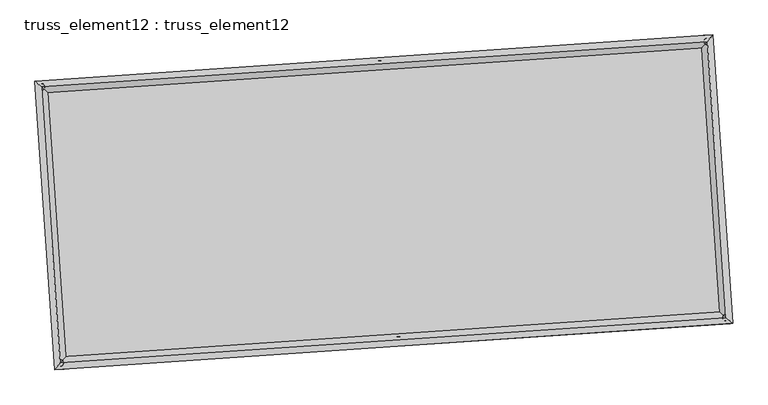
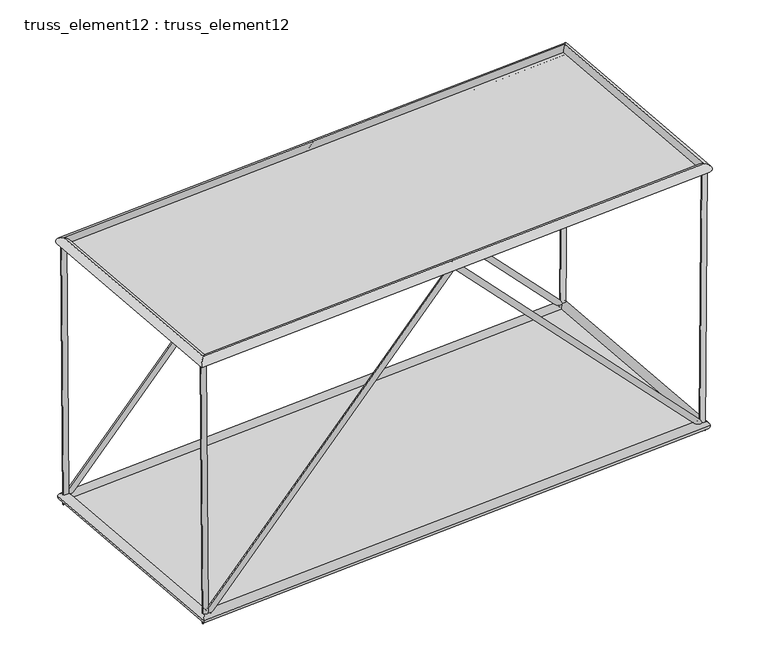
"""IFC4 building model written with IfcOpenShell, lengths in millimetres: plate geometry, truss_element12 : truss_element12."""

import ifcopenshell
import ifcopenshell.guid

model = None  # the IFC model being written
_history = None  # IfcOwnerHistory: only IFC2X3 demands one
_inside = {}  # id of a spatial element -> (the spatial element, [elements in it])
_under = {}  # id of a project, library or spatial element -> (it, [spatial elements below it])
_declared = {}  # id of a project -> (the project, [libraries it declares])
_typed = {}  # id of a type object -> (the type object, [elements of that type])
_made_of = {}  # id of a material, layer set ... -> (it, [elements and type objects made of it])


def new_model(schema):
    """Start an empty IFC model of exactly this schema.

    Asked for "IFC4X3", IfcOpenShell would pick the latest addendum, in which some entities
    have other attributes; the version numbers below select the first issue.
    IFC2X3 requires an IfcOwnerHistory on every rooted entity: one is made here for all.
    """
    global model, _history
    if schema == "IFC4X3":
        model = ifcopenshell.file(schema_version=(4, 3, 0, 0))
    else:
        model = ifcopenshell.file(schema=schema)
    _inside.clear()
    _under.clear()
    _declared.clear()
    _typed.clear()
    _made_of.clear()
    _history = None
    if model.schema == "IFC2X3":
        org = make("IfcOrganization", Name="unknown")
        user = make(
            "IfcPersonAndOrganization",
            ThePerson=make("IfcPerson", FamilyName="unknown"),
            TheOrganization=org,
        )
        app = make(
            "IfcApplication",
            ApplicationDeveloper=org,
            Version="unknown",
            ApplicationFullName="unknown",
            ApplicationIdentifier="unknown",
        )
        _history = make(
            "IfcOwnerHistory",
            OwningUser=user,
            OwningApplication=app,
            ChangeAction="ADDED",
            CreationDate=0,
        )
    return model


def make(cls, **values):
    """One entity of the class cls with the attributes given. An attribute that is None is left unset."""
    return model.create_entity(
        cls, **{name: value for name, value in values.items() if value is not None}
    )


def rooted(cls, **values):
    """An entity with a GlobalId (a new one), such as an element, a storey or a relation."""
    return make(cls, GlobalId=ifcopenshell.guid.new(), OwnerHistory=_history, **values)


def si_unit(unit_type, name, prefix=None):
    """IfcSIUnit, for example si_unit("LENGTHUNIT", "METRE", prefix="MILLI")."""
    return make("IfcSIUnit", UnitType=unit_type, Prefix=prefix, Name=name)


def assignment(units):
    """IfcUnitAssignment: the units of a project."""
    return None if units is None else make("IfcUnitAssignment", Units=units)


def point(xyz):
    """IfcCartesianPoint."""
    return None if xyz is None else make("IfcCartesianPoint", Coordinates=xyz)


def direction(xyz):
    """IfcDirection."""
    return None if xyz is None else make("IfcDirection", DirectionRatios=xyz)


def frame(location, z_axis=None, x_axis=None):
    """IfcAxis2Placement3D, a coordinate frame: its origin and axes. An axis left out is left unset."""
    return make(
        "IfcAxis2Placement3D",
        Location=point(location),
        Axis=direction(z_axis),
        RefDirection=direction(x_axis),
    )


def origin():
    """The frame at (0, 0, 0) with its axes left unset."""
    return frame((0.0, 0.0, 0.0))


def origin_with_axes():
    """The frame at (0, 0, 0) with the z axis (0, 0, 1) and the x axis (1, 0, 0) written out."""
    return frame((0.0, 0.0, 0.0), z_axis=(0.0, 0.0, 1.0), x_axis=(1.0, 0.0, 0.0))


def place(relative_to, where):
    """IfcLocalPlacement: puts the frame where relative to a parent placement (None: the world)."""
    return make(
        "IfcLocalPlacement", PlacementRelTo=relative_to, RelativePlacement=where
    )


def context(
    kind, dimensions, precision=None, world=None, true_north=None, identifier=None
):
    """IfcGeometricRepresentationContext, for example the 3D "Model" context."""
    return make(
        "IfcGeometricRepresentationContext",
        ContextIdentifier=identifier,
        ContextType=kind,
        CoordinateSpaceDimension=dimensions,
        Precision=precision,
        WorldCoordinateSystem=world,
        TrueNorth=true_north,
    )


def project(units=None, contexts=None):
    """IfcProject with its units and contexts."""
    return rooted(
        "IfcProject",
        Name="project",
        RepresentationContexts=contexts,
        UnitsInContext=assignment(units),
    )


def spatial(cls, under=None, at=None, **own):
    """A site, building, storey or space (cls), placed at a placement, below another one or the project."""
    s = rooted(cls, ObjectPlacement=at, **own)
    if under is not None:
        _under.setdefault(under.id(), (under, []))[1].append(s)
    return s


def polyline(points):
    """IfcPolyline through the points."""
    return make("IfcPolyline", Points=[point(p) for p in points])


def circle_curve(where, radius):
    """IfcCircle in the frame where."""
    return make("IfcCircle", Position=where, Radius=radius)


def ellipse_curve(where, semi_axis1, semi_axis2):
    """IfcEllipse in the frame where."""
    return make(
        "IfcEllipse", Position=where, SemiAxis1=semi_axis1, SemiAxis2=semi_axis2
    )


def outline(outer, holes=None, kind="AREA"):
    """IfcArbitraryClosedProfileDef: a profile drawn as a closed curve; with holes, ...WithVoids."""
    if holes is None:
        return make("IfcArbitraryClosedProfileDef", ProfileType=kind, OuterCurve=outer)
    return make(
        "IfcArbitraryProfileDefWithVoids",
        ProfileType=kind,
        OuterCurve=outer,
        InnerCurves=holes,
    )


def extrude(swept, where, along, depth):
    """IfcExtrudedAreaSolid: the profile swept, set in the frame where, extruded along a direction by depth."""
    return make(
        "IfcExtrudedAreaSolid",
        SweptArea=swept,
        Position=where,
        ExtrudedDirection=direction(along),
        Depth=depth,
    )


def shape(context_of_items, identifier, shape_type, items):
    """IfcShapeRepresentation: the items that make up one representation, for example the "Body"."""
    return make(
        "IfcShapeRepresentation",
        ContextOfItems=context_of_items,
        RepresentationIdentifier=identifier,
        RepresentationType=shape_type,
        Items=items,
    )


def source(mapping_origin, context_of_items, identifier, shape_type, items):
    """IfcRepresentationMap: a shape defined once, which mapped items show again and again."""
    return make(
        "IfcRepresentationMap",
        MappingOrigin=mapping_origin,
        MappedRepresentation=shape(context_of_items, identifier, shape_type, items),
    )


def transform(
    local_origin,
    x_axis=None,
    y_axis=None,
    z_axis=None,
    scale=None,
    scale2=None,
    scale3=None,
    uniform=True,
):
    """IfcCartesianTransformationOperator3D, or its non-uniform kind. x_axis, y_axis, z_axis: its Axis1, 2, 3."""
    if uniform:
        return make(
            "IfcCartesianTransformationOperator3D",
            Axis1=direction(x_axis),
            Axis2=direction(y_axis),
            LocalOrigin=point(local_origin),
            Scale=scale,
            Axis3=direction(z_axis),
        )
    return make(
        "IfcCartesianTransformationOperator3DnonUniform",
        Axis1=direction(x_axis),
        Axis2=direction(y_axis),
        LocalOrigin=point(local_origin),
        Scale=scale,
        Axis3=direction(z_axis),
        Scale2=scale2,
        Scale3=scale3,
    )


def mapped(mapping_source, mapping_target):
    """IfcMappedItem: shows the shape of a source again, moved by a transform."""
    return make(
        "IfcMappedItem", MappingSource=mapping_source, MappingTarget=mapping_target
    )


def made_of(thing, what):
    """Note that an element or type object is made of a material, layer set ...; save() writes the relation."""
    if what is not None:
        _made_of.setdefault(what.id(), (what, []))[1].append(thing)
    return thing


def element(
    cls,
    number,
    at=None,
    inside=None,
    cuts=None,
    type_object=None,
    material=None,
    context=None,
    identifier="Body",
    shape_type=None,
    held_by="IfcProductDefinitionShape",
    body=None,
    shapes=None,
    **own,
):
    """One element of the class cls, such as IfcWall. Its Tag is "e" and its number.

    at: its placement. inside: the storey or other place that contains it. cuts: it is an
    opening in that element (IfcRelVoidsElement). A single representation is given by context,
    identifier, shape_type and body (its items); several are given by shapes. held_by: the class
    of the entity that holds the representations. save() writes the other relations.
    """
    e = rooted(cls, Tag="e%d" % number, ObjectPlacement=at, **own)
    if body is not None:
        shapes = [shape(context, identifier, shape_type, body)]
    if shapes is not None:
        e.Representation = make(held_by, Representations=shapes)
    if inside is not None:
        _inside.setdefault(inside.id(), (inside, []))[1].append(e)
    if cuts is not None:
        rooted(
            "IfcRelVoidsElement", RelatingBuildingElement=cuts, RelatedOpeningElement=e
        )
    if type_object is not None:
        _typed.setdefault(type_object.id(), (type_object, []))[1].append(e)
    return made_of(e, material)


def aggregate(whole, parts):
    """IfcRelAggregates: a whole, such as a stair, and the parts it consists of."""
    return rooted("IfcRelAggregates", RelatingObject=whole, RelatedObjects=parts)


def save(model, path):
    """Write the relations noted so far, then the file.

    IfcRelAggregates (storeys below a building ...), IfcRelContainedInSpatialStructure (elements
    in a storey), IfcRelDefinesByType, IfcRelAssociatesMaterial and IfcRelDeclares: one each for
    every whole, place, type object, material and project.
    """
    for whole, parts in _under.values():
        aggregate(whole, parts)
    for where, things in _inside.values():
        rooted(
            "IfcRelContainedInSpatialStructure",
            RelatedElements=things,
            RelatingStructure=where,
        )
    for kind, things in _typed.values():
        rooted("IfcRelDefinesByType", RelatedObjects=things, RelatingType=kind)
    for what, things in _made_of.values():
        rooted("IfcRelAssociatesMaterial", RelatedObjects=things, RelatingMaterial=what)
    for by, libraries in _declared.values():
        rooted("IfcRelDeclares", RelatingContext=by, RelatedDefinitions=libraries)
    model.write(path)


def plane_surface(at):
    """IfcPlane: the flat surface through the origin of the frame at, square to its z axis."""
    return make("IfcPlane", Position=at)


def cylinder_surface(at, radius):
    """IfcCylindricalSurface: all points at the distance radius from the z axis of the frame at."""
    return make("IfcCylindricalSurface", Position=at, Radius=radius)


def advanced_brep(points, edges, surfaces, faces):
    """IfcAdvancedBrep: a solid bounded by faces that lie on surfaces and meet in shared edges.

    An edge is (start, end): straight between two places in points (the first is 0);
    or (start, end, curve); or (start, end, curve, False) where it runs against its curve.
    A face is (place in surfaces, loops), or (place, loops, False) where it looks against
    its surface's normal. A loop lists edges by number (the first is 1), with a minus sign
    where the edge is run from its end to its start. The first loop is the outer one.
    """
    corners = [point(p) for p in points]
    vertices = [make("IfcVertexPoint", VertexGeometry=c) for c in corners]
    made = []
    for start, end, *more in edges:
        made.append(
            make(
                "IfcEdgeCurve",
                EdgeStart=vertices[start],
                EdgeEnd=vertices[end],
                EdgeGeometry=more[0] if more else make("IfcPolyline", Points=[corners[start], corners[end]]),
                SameSense=more[1] if len(more) > 1 else True,
            )
        )
    hull = []
    for where, loops, *sense in faces:
        bounds = []
        for j, loop in enumerate(loops):
            ring = [make("IfcOrientedEdge", EdgeElement=made[abs(k) - 1], Orientation=k > 0) for k in loop]
            bounds.append(
                make(
                    "IfcFaceOuterBound" if j == 0 else "IfcFaceBound",
                    Bound=make("IfcEdgeLoop", EdgeList=ring),
                    Orientation=True,
                )
            )
        hull.append(make("IfcAdvancedFace", Bounds=bounds, FaceSurface=surfaces[where], SameSense=sense[0] if sense else True))
    return make("IfcAdvancedBrep", Outer=make("IfcClosedShell", CfsFaces=hull))


def truss_element12_truss_element12_81932074(model_context):
    return source(origin(), model_context, "Body", "SolidModel", [
        advanced_brep(
        [(-3702.688172, 2273.6501932, 5000.2343714), (-3801.788684, 2260.2891126, 4999.4793629), (-3665.8706913, 2276.1606372, 123.2387715), (-3763.1161915, 2262.9260429, -123.2387715), (1063.4172149, 2598.6328018, 5071.9820194), (1063.8699312, 2592.0598775, 4927.7362286), (5793.2948238, 2921.145176, 123.2430249), (5891.4661532, 2921.2353125, -123.2430249), (5829.5270694, 2923.6157151, 5000.2328852), (5929.5240788, 2923.8303377, 4999.4898764)],
        [
            (0, 1, circle_curve(frame((-3752.238428, 2266.9696529, 4999.8568672), z_axis=(-0.007548997314577087, -0.000514737430455595, 0.999971373432721), x_axis=(-0.13361086689497337, 0.9910337470163174, -0.0004985201818760374)), 50.0)),
            (1, 0, circle_curve(frame((-3752.238428, 2266.9696529, 4999.8568672), z_axis=(-0.007548997314577087, -0.000514737430455595, 0.999971373432721), x_axis=(-0.13361086689497337, 0.9910337470163174, -0.0004985201818760374)), 50.0)),
            (0, 2),
            (2, 3, ellipse_curve(frame((-3714.4934414, 2269.54334, 0.0), z_axis=(-0.9271929359308112, -0.06322176171080186, 0.36921033084975474), x_axis=(0.36835501674811216, 0.025116728343544507, 0.9293458622029878)), 132.8968359, 50.0)),
            (3, 1),
            (3, 2, ellipse_curve(frame((-3714.4934414, 2269.54334, 0.0), z_axis=(-0.9271929359308112, -0.06322176171080186, 0.36921033084975474), x_axis=(0.36835501674811216, 0.025116728343544507, 0.9293458622029878)), 132.8968359, 50.0)),
            (2, 4),
            (4, 5, ellipse_curve(frame((1063.6435731, 2595.3463397, 4999.859124), z_axis=(-0.9976833955843888, -0.06802823819525586, -3.135687396447292e-05), x_axis=(3.12842325072798e-05, 2.133152891987861e-06, -0.9999999995083733)), 72.2799434, 50.0)),
            (5, 3),
            (5, 4, ellipse_curve(frame((1063.6435731, 2595.3463397, 4999.859124), z_axis=(-0.9976833955843888, -0.06802823819525586, -3.135687396447292e-05), x_axis=(3.12842325072798e-05, 2.133152891987861e-06, -0.9999999995083733)), 72.2799434, 50.0)),
            (4, 6),
            (6, 7, ellipse_curve(frame((5842.3804885, 2921.1902443, 0.0), z_axis=(-0.9271592320010842, -0.06321946356795421, -0.36929535326258833), x_axis=(-0.36843984219769044, -0.025122512268499313, 0.9293120800133075)), 132.9062538, 50.0)),
            (7, 5),
            (7, 6, ellipse_curve(frame((5842.3804885, 2921.1902443, 0.0), z_axis=(-0.9271592320010842, -0.06321946356795421, -0.36929535326258833), x_axis=(-0.36843984219769044, -0.025122512268499313, 0.9293120800133075)), 132.9062538, 50.0)),
            (8, 9, circle_curve(frame((5879.5255741, 2923.7230264, 4999.8613808), z_axis=(0.007429017120522426, 0.0005065564371105527, 0.9999722761682942), x_axis=(-0.0021499302803911083, 0.999997568554261, -0.0004905969378120464)), 50.0)),
            (9, 8, circle_curve(frame((5879.5255741, 2923.7230264, 4999.8613808), z_axis=(0.007429017120522426, 0.0005065564371105527, 0.9999722761682942), x_axis=(-0.0021499302803911083, 0.999997568554261, -0.0004905969378120464)), 50.0)),
            (6, 8),
            (9, 7),
        ],
        [
            plane_surface(frame((-3752.238428, 2316.9696463, 4999.8826048), z_axis=(-0.007548997314575647, -0.0005147374304560255, 0.9999713734327211), x_axis=(0.9999715059138159, -3.885862204455747e-06, 0.007548996314447718))),
            cylinder_surface(frame((-3752.238428, 2266.9696529, 4999.8568672), z_axis=(-0.007548997314577087, -0.000514737430455595, 0.999971373432721), x_axis=(-0.13361086689497337, 0.9910337470163174, -0.0004985201818760374)), 50.0),
            cylinder_surface(frame((-3714.4934414, 2269.54334, 0.0), z_axis=(-0.6901297168790946, -0.04705732196532738, -0.7221541264368931), x_axis=(-0.02041156189161515, 0.9987523773136525, -0.04557474027871566)), 50.0),
            cylinder_surface(frame((1063.6435731, 2595.3463397, 4999.859124), z_axis=(-0.6901748995971223, -0.04706040280311382, 0.7221107438988223), x_axis=(-0.115346442987764, 0.9922791286529746, -0.04557772405203943)), 50.0),
            plane_surface(frame((5879.5255741, 2873.7230329, 4999.8867094), z_axis=(0.007429017120522355, 0.0005065564371127904, 0.9999722761682942), x_axis=(0.999972404471555, -3.7633202953912764e-06, -0.0074290161673289294))),
            cylinder_surface(frame((5842.3804885, 2921.1902443, 0.0), z_axis=(-0.007429017120522424, -0.0005065564371105526, -0.999972276168294), x_axis=(-0.0021499302803911083, 0.999997568554261, -0.0004905969378120464)), 50.0),
        ],
        [
            (0, [[1, 2]]),
            (1, [[-1, 3, 4, 5]]),
            (1, [[-2, -5, 6, -3]]),
            (2, [[-4, 7, 8, 9]]),
            (2, [[-6, -9, 10, -7]]),
            (3, [[-8, 11, 12, 13]]),
            (3, [[-10, -13, 14, -11]]),
            (4, [[15, 16]]),
            (5, [[-12, 17, -16, 18]]),
            (5, [[-14, -18, -15, -17]]),
        ],
    ),
        advanced_brep(
        [(-3430.575219, -1717.0833911, 5000.2343714), (-3529.6757311, -1730.4444717, 4999.4793629), (-3393.7577384, -1714.5729471, 123.2387715), (-3491.0032386, -1727.8075414, -123.2387715), (1335.5301678, -1392.1007825, 5071.9820194), (1335.9828841, -1398.6737068, 4927.7362286), (6065.4077767, -1069.5884083, 123.2430249), (6163.5791061, -1069.4982718, -123.2430249), (6101.6400224, -1067.1178692, 5000.2328852), (6201.6370317, -1066.9032466, 4999.4898764)],
        [
            (0, 1, circle_curve(frame((-3480.1254751, -1723.7639314, 4999.8568672), z_axis=(-0.00754899731457709, -0.0005147374304555873, 0.999971373432721), x_axis=(-0.13361086689497323, 0.9910337470163173, -0.0004985201818760446)), 50.0)),
            (1, 0, circle_curve(frame((-3480.1254751, -1723.7639314, 4999.8568672), z_axis=(-0.00754899731457709, -0.0005147374304555873, 0.999971373432721), x_axis=(-0.13361086689497323, 0.9910337470163173, -0.0004985201818760446)), 50.0)),
            (0, 2),
            (2, 3, ellipse_curve(frame((-3442.3804885, -1721.1902443, 0.0), z_axis=(-0.9271929359308112, -0.06322176171080175, 0.3692103308497547), x_axis=(0.3683550167481121, 0.025116728343544472, 0.9293458622029878)), 132.8968359, 50.0)),
            (3, 1),
            (3, 2, ellipse_curve(frame((-3442.3804885, -1721.1902443, 0.0), z_axis=(-0.9271929359308112, -0.06322176171080175, 0.3692103308497547), x_axis=(0.3683550167481121, 0.025116728343544472, 0.9293458622029878)), 132.8968359, 50.0)),
            (2, 4),
            (4, 5, ellipse_curve(frame((1335.756526, -1395.3872446, 4999.859124), z_axis=(-0.9976833955843888, -0.06802823819525583, -3.135687396431242e-05), x_axis=(3.1284232507126054e-05, 2.1331528920551236e-06, -0.9999999995083733)), 72.2799434, 50.0)),
            (5, 3),
            (5, 4, ellipse_curve(frame((1335.756526, -1395.3872446, 4999.859124), z_axis=(-0.9976833955843888, -0.06802823819525583, -3.135687396431242e-05), x_axis=(3.1284232507126054e-05, 2.1331528920551236e-06, -0.9999999995083733)), 72.2799434, 50.0)),
            (4, 6),
            (6, 7, ellipse_curve(frame((6114.4934414, -1069.54334, 0.0), z_axis=(-0.9271592320010842, -0.06321946356795434, -0.3692953532625882), x_axis=(-0.3684398421976903, -0.025122512268499313, 0.9293120800133076)), 132.9062538, 50.0)),
            (7, 5),
            (7, 6, ellipse_curve(frame((6114.4934414, -1069.54334, 0.0), z_axis=(-0.9271592320010842, -0.06321946356795434, -0.3692953532625882), x_axis=(-0.3684398421976903, -0.025122512268499313, 0.9293120800133076)), 132.9062538, 50.0)),
            (8, 9, circle_curve(frame((6151.638527, -1067.0105579, 4999.8613808), z_axis=(0.0074290171205225845, 0.0005065564371106023, 0.9999722761682942), x_axis=(-0.002149930280391232, 0.999997568554261, -0.0004905969378120946)), 50.0)),
            (9, 8, circle_curve(frame((6151.638527, -1067.0105579, 4999.8613808), z_axis=(0.0074290171205225845, 0.0005065564371106023, 0.9999722761682942), x_axis=(-0.002149930280391232, 0.999997568554261, -0.0004905969378120946)), 50.0)),
            (6, 8),
            (9, 7),
        ],
        [
            plane_surface(frame((-3480.1254751, -1673.763938, 4999.8826048), z_axis=(-0.007548997314575647, -0.0005147374304560255, 0.9999713734327211), x_axis=(0.9999715059138159, -3.885862204455747e-06, 0.007548996314447718))),
            cylinder_surface(frame((-3480.1254751, -1723.7639314, 4999.8568672), z_axis=(-0.00754899731457709, -0.0005147374304555873, 0.999971373432721), x_axis=(-0.13361086689497323, 0.9910337470163173, -0.0004985201818760446)), 50.0),
            cylinder_surface(frame((-3442.3804885, -1721.1902443, 0.0), z_axis=(-0.6901297168790949, -0.047057321965327324, -0.722154126436893), x_axis=(-0.020411561891615058, 0.9987523773136525, -0.04557474027871568)), 50.0),
            cylinder_surface(frame((1335.756526, -1395.3872446, 4999.859124), z_axis=(-0.6901748995971222, -0.04706040280311387, 0.7221107438988226), x_axis=(-0.11534644298776417, 0.9922791286529747, -0.04557772405203947)), 50.0),
            plane_surface(frame((6151.638527, -1117.0105514, 4999.8867094), z_axis=(0.007429017120522355, 0.0005065564371127918, 0.9999722761682942), x_axis=(0.999972404471555, -3.763320294503098e-06, -0.0074290161673289294))),
            cylinder_surface(frame((6114.4934414, -1069.54334, 0.0), z_axis=(-0.007429017120522583, -0.0005065564371106022, -0.999972276168294), x_axis=(-0.002149930280391232, 0.999997568554261, -0.0004905969378120946)), 50.0),
        ],
        [
            (0, [[1, 2]]),
            (1, [[-1, 3, 4, 5]]),
            (1, [[-2, -5, 6, -3]]),
            (2, [[-4, 7, 8, 9]]),
            (2, [[-6, -9, 10, -7]]),
            (3, [[-8, 11, 12, 13]]),
            (3, [[-10, -13, 14, -11]]),
            (4, [[15, 16]]),
            (5, [[-12, 17, -16, 18]]),
            (5, [[-14, -18, -15, -17]]),
        ],
    ),
        advanced_brep(
        [(-3480.1242844, -1723.7626117, 4909.8568672), (-3480.1266658, -1723.7652511, 5089.8568672), (-3752.2397868, 2266.9707988, 5089.8568672), (-3752.2370692, 2266.968507, 4909.8568672), (5879.5266809, 2923.7243404, 5089.8613808), (5879.5244674, 2923.7217124, 4909.8613808), (6151.6398019, -1067.0117095, 5089.8613808), (6151.6372521, -1067.0094063, 4909.8613808)],
        [
            (0, 1, ellipse_curve(frame((-3480.1254751, -1723.7639314, 4999.8568672), z_axis=(-0.7535719234053797, 0.6573654662780873, -3.3059971506810466e-07), x_axis=(-0.657365466278005, -0.7535719234054516, -3.305997150681247e-07)), 127.2792206, 90.0)),
            (1, 2),
            (2, 3, ellipse_curve(frame((-3752.238428, 2266.9696529, 4999.8568672), z_axis=(-0.657365466278005, -0.7535719234054515, -3.3059971506814293e-07), x_axis=(0.7535719234053796, -0.6573654662780875, 3.3059971506812287e-07)), 127.2792206, 90.0)),
            (3, 0),
            (1, 0, ellipse_curve(frame((-3480.1254751, -1723.7639314, 4999.8568672), z_axis=(-0.7535719234053797, 0.6573654662780873, -3.3059971506810466e-07), x_axis=(-0.657365466278005, -0.7535719234054516, -3.305997150681247e-07)), 127.2792206, 90.0)),
            (3, 2, ellipse_curve(frame((-3752.238428, 2266.9696529, 4999.8568672), z_axis=(-0.657365466278005, -0.7535719234054515, -3.3059971506814293e-07), x_axis=(0.7535719234053796, -0.6573654662780875, 3.3059971506812287e-07)), 127.2792206, 90.0)),
            (2, 4),
            (4, 5, ellipse_curve(frame((5879.5255741, 2923.7230264, 4999.8613808), z_axis=(-0.7535719234053798, 0.6573654662780873, -3.3059971506814087e-07), x_axis=(-0.657365466278005, -0.7535719234054515, -3.30599715068125e-07)), 127.2792206, 90.0)),
            (5, 3),
            (5, 4, ellipse_curve(frame((5879.5255741, 2923.7230264, 4999.8613808), z_axis=(-0.7535719234053798, 0.6573654662780873, -3.3059971506814087e-07), x_axis=(-0.657365466278005, -0.7535719234054515, -3.30599715068125e-07)), 127.2792206, 90.0)),
            (4, 6),
            (6, 7, ellipse_curve(frame((6151.638527, -1067.0105579, 4999.8613808), z_axis=(0.657365466278005, 0.7535719234054516, 3.305997150681068e-07), x_axis=(-0.7535719234053797, 0.6573654662780875, -3.305997150681227e-07)), 127.2792206, 90.0)),
            (7, 5),
            (7, 6, ellipse_curve(frame((6151.638527, -1067.0105579, 4999.8613808), z_axis=(0.657365466278005, 0.7535719234054516, 3.305997150681068e-07), x_axis=(-0.7535719234053797, 0.6573654662780875, -3.305997150681227e-07)), 127.2792206, 90.0)),
            (6, 1),
            (0, 7),
        ],
        [
            cylinder_surface(frame((-3480.1254751, -1723.7639314, 4999.8568672), z_axis=(0.06802823822870085, -0.9976833960748767, 0.0), x_axis=(-0.9976833959743321, -0.0680282382218451, -1.4197044524281848e-05)), 90.0),
            cylinder_surface(frame((-3752.238428, 2266.9696529, 4999.8568672), z_axis=(-0.9976833960747679, -0.0680282382286909, -4.675386007660345e-07), x_axis=(-0.0680282382158825, 0.9976833959812822, -1.3729505923559892e-05)), 90.0),
            cylinder_surface(frame((5879.5255741, 2923.7230264, 4999.8613808), z_axis=(-0.0680282382287009, 0.9976833960748767, 0.0), x_axis=(0.9976833959871405, 0.0680282382227185, -1.3261967322837937e-05)), 90.0),
            cylinder_surface(frame((6151.638527, -1067.0105579, 4999.8613808), z_axis=(0.9976833960747677, 0.06802823822869078, 4.675386007660087e-07), x_axis=(0.06802823822869078, -0.9976833959804088, -1.3729505923559892e-05)), 90.0),
        ],
        [
            (0, [[1, 2, 3, 4]]),
            (0, [[5, -4, 6, -2]]),
            (1, [[-3, 7, 8, 9]]),
            (1, [[-6, -9, 10, -7]]),
            (2, [[-8, 11, 12, 13]]),
            (2, [[-10, -13, 14, -11]]),
            (3, [[-12, 15, -1, 16]]),
            (3, [[-14, -16, -5, -15]]),
        ],
    ),
        advanced_brep(
        [(-3358.7115243, -1625.2761972, 0.0), (-3526.0494527, -1817.1042913, 0.0), (-3810.4074885, 2353.2123043, 0.0), (-3618.5793943, 2185.8743758, 0.0), (5926.0494527, 3017.1042913, 0.0), (5758.7115243, 2825.2761972, 0.0), (6210.4074885, -1153.2123043, 0.0), (6018.5793943, -985.8743758, 0.0)],
        [
            (0, 1, ellipse_curve(frame((-3442.3804885, -1721.1902443, 0.0), z_axis=(-0.7535719234054581, 0.6573654662780807, 0.0), x_axis=(-0.6573654662780808, -0.7535719234054581, 0.0)), 127.2792206, 90.0)),
            (1, 2),
            (2, 3, ellipse_curve(frame((-3714.4934414, 2269.54334, 0.0), z_axis=(-0.6573654662780807, -0.753571923405458, 0.0), x_axis=(0.7535719234054579, -0.6573654662780808, 0.0)), 127.2792206, 90.0)),
            (3, 0),
            (1, 0, ellipse_curve(frame((-3442.3804885, -1721.1902443, 0.0), z_axis=(-0.7535719234054581, 0.6573654662780807, 0.0), x_axis=(-0.6573654662780808, -0.7535719234054581, 0.0)), 127.2792206, 90.0)),
            (3, 2, ellipse_curve(frame((-3714.4934414, 2269.54334, 0.0), z_axis=(-0.6573654662780807, -0.753571923405458, 0.0), x_axis=(0.7535719234054579, -0.6573654662780808, 0.0)), 127.2792206, 90.0)),
            (2, 4),
            (4, 5, ellipse_curve(frame((5842.3804885, 2921.1902443, 0.0), z_axis=(-0.7535719234054582, 0.6573654662780806, 0.0), x_axis=(-0.6573654662780805, -0.7535719234054583, 0.0)), 127.2792206, 90.0)),
            (5, 3),
            (5, 4, ellipse_curve(frame((5842.3804885, 2921.1902443, 0.0), z_axis=(-0.7535719234054582, 0.6573654662780806, 0.0), x_axis=(-0.6573654662780805, -0.7535719234054583, 0.0)), 127.2792206, 90.0)),
            (4, 6),
            (6, 7, ellipse_curve(frame((6114.4934414, -1069.54334, 0.0), z_axis=(0.6573654662780806, 0.7535719234054581, 0.0), x_axis=(-0.7535719234054581, 0.6573654662780806, 0.0)), 127.2792206, 90.0)),
            (7, 5),
            (7, 6, ellipse_curve(frame((6114.4934414, -1069.54334, 0.0), z_axis=(0.6573654662780806, 0.7535719234054581, 0.0), x_axis=(-0.7535719234054581, 0.6573654662780806, 0.0)), 127.2792206, 90.0)),
            (6, 1),
            (0, 7),
        ],
        [
            cylinder_surface(frame((-3442.3804885, -1721.1902443, 0.0), z_axis=(0.06802823822870274, -0.9976833960748764, 0.0), x_axis=(-0.9976833960748764, -0.06802823822870274, 0.0)), 90.0),
            cylinder_surface(frame((-3714.4934414, 2269.54334, 0.0), z_axis=(-0.9976833960748767, -0.06802823822870008, 0.0), x_axis=(-0.06802823822870008, 0.9976833960748767, 0.0)), 90.0),
            cylinder_surface(frame((5842.3804885, 2921.1902443, 0.0), z_axis=(-0.06802823822870283, 0.9976833960748764, 0.0), x_axis=(0.9976833960748764, 0.06802823822870283, 0.0)), 90.0),
            cylinder_surface(frame((6114.4934414, -1069.54334, 0.0), z_axis=(0.9976833960748767, 0.06802823822870016, 0.0), x_axis=(0.06802823822870016, -0.9976833960748767, 0.0)), 90.0),
        ],
        [
            (0, [[1, 2, 3, 4]]),
            (0, [[5, -4, 6, -2]]),
            (1, [[-3, 7, 8, 9]]),
            (1, [[-6, -9, 10, -7]]),
            (2, [[-8, 11, 12, 13]]),
            (2, [[-10, -13, 14, -11]]),
            (3, [[-12, 15, -1, 16]]),
            (3, [[-14, -16, -5, -15]]),
        ],
    ),
        extrude(outline(polyline([(-3442.3804885, -1721.1902443), (-3714.4934414, 2269.54334), (5842.3804885, 2921.1902443), (6114.4934414, -1069.54334), (-3442.3804885, -1721.1902443)])), origin_with_axes(), (0.0, 0.0, 1.0), 20.0),
        extrude(outline(polyline([(-2000.0, 4827.0643974), (2000.0, 4827.0643974), (2000.0, -4827.0643974), (-2000.0, -4827.0643974), (-2000.0, 4827.0643974)])), frame((1199.7000495, 599.9795475, 4999.859124), z_axis=(-4.6645549900834067e-07, -3.180582731402529e-08, 0.9999999999998909), x_axis=(-0.06802823822870274, 0.9976833960748764, 0.0)), (0.0, 0.0, 1.0), 20.0),
    ])


if __name__ == "__main__":
    model = new_model("IFC4")
    model_context = context("Model", 3, world=origin())
    ifc_project = project(units=[si_unit("LENGTHUNIT", "METRE", prefix="MILLI")], contexts=[model_context])
    site = spatial("IfcSite", under=ifc_project)
    building = spatial("IfcBuilding", under=site)
    placement = place(None, origin())
    truss_element12_truss_element12_shape = truss_element12_truss_element12_81932074(model_context)
    element("IfcPlate", 1, ObjectType="truss_element12 : truss_element12", at=placement, inside=building, context=model_context, shape_type="MappedRepresentation", body=[
        mapped(truss_element12_truss_element12_shape, transform((0.0, 0.0, 0.0), x_axis=(1.0, 0.0, 0.0), y_axis=(0.0, 1.0, 0.0), z_axis=(0.0, 0.0, 1.0))),
    ])
    save(model, "model.ifc")

# Revit data of these elements
# Type "truss_element12 : truss_element12"
#   steellbar1 = 90 mm
#   steelbar2 = 50 mm
#   offset1 = 5000 mm
#   M = Default Roof
# Element 1 (IfcPlate, "truss_element12 : truss_element12")
#   Materials on its faces: "Default Roof"
# Materials
#   "Default Roof": class "Miscellaneous", colour RGB 0 127 0, transparency 0, Comments = "Rendering appearance not upgraded Rendering appearance not upgraded ", Cost = 0
